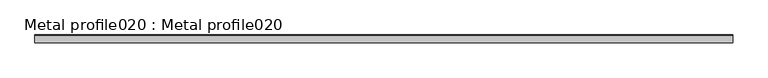
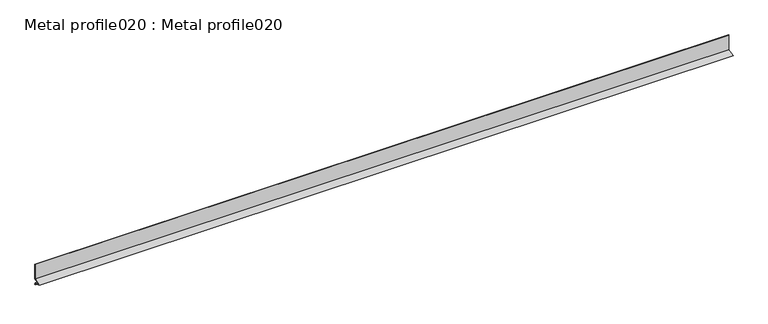
"""IFC4 building model written with IfcOpenShell, lengths in millimetres: proxy geometry, Metal profile020 : Metal profile020."""

from ifc_helpers import new_model, si_unit, frame, origin, place, context, project, spatial, polyline, outline, extrude, source, transform, mapped, element, save


def metal_profile020_metal_profile020_ed83d00a(model_context):
    return source(origin(), model_context, "Body", "SweptSolid", [
        extrude(outline(polyline([(-4418.7737868, 40296.1778532), (-4420.0218493, 40295.9428216), (-4420.8451703, 40300.3148134), (-4440.9987868, 40306.7927615), (-4420.0437868, 40313.5282972), (-4420.0437868, 40357.5927615), (-4418.7737868, 40357.5927615), (-4418.7737868, 40312.6025179), (-4436.8485845, 40306.7927615), (-4419.7369819, 40301.2926035), (-4418.7737868, 40296.1778532)])), frame((12383.0178845, 0.0, 0.0), z_axis=(1.0, 0.0, 0.0), x_axis=(0.0, 1.0, 0.0)), (0.0, 0.0, 1.0), 2000.0),
    ])


if __name__ == "__main__":
    model = new_model("IFC4")
    model_context = context("Model", 3, world=origin())
    ifc_project = project(units=[si_unit("LENGTHUNIT", "METRE", prefix="MILLI")], contexts=[model_context])
    site = spatial("IfcSite", under=ifc_project)
    building = spatial("IfcBuilding", under=site)
    placement = place(None, origin())
    metal_profile020_metal_profile020_shape = metal_profile020_metal_profile020_ed83d00a(model_context)
    element("IfcBuildingElementProxy", 1, Name="Metal profile020 : Metal profile020", ObjectType="Metal profile020 : Metal profile020", at=placement, inside=building, context=model_context, shape_type="MappedRepresentation", body=[
        mapped(metal_profile020_metal_profile020_shape, transform((0.0, 0.0, 0.0), x_axis=(1.0, 0.0, 0.0), y_axis=(0.0, 1.0, 0.0), z_axis=(0.0, 0.0, 1.0))),
    ])
    save(model, "model.ifc")

# Revit data of these elements
# Type "Metal profile020 : Metal profile020"
#   NameOverride = "Metal profile020"
# Element 1 (IfcBuildingElementProxy, "Metal profile020 : Metal profile020")
#   Materials on its faces: "16 GA. COPPER WEEP SCREED W/ MIN 3 1/2\" ATTACHMENT FLANGE - LAP UNDERLAYMENT OVER WEED SCREED"
# Materials
#   "16 GA. COPPER WEEP SCREED W/ MIN 3 1/2\" ATTACHMENT FLANGE - LAP UNDERLAYMENT OVER WEED SCREED": class "Unassigned", colour RGB 251 232 155, transparency 0, Cost = 0
